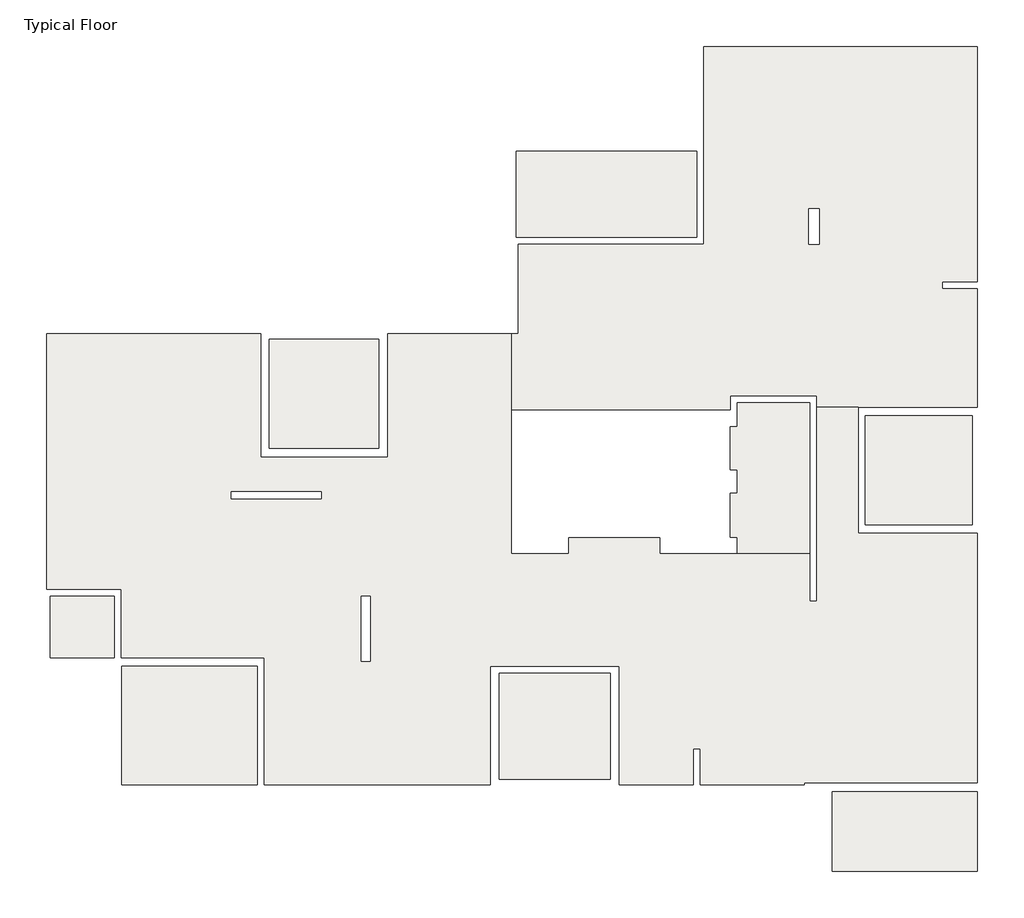
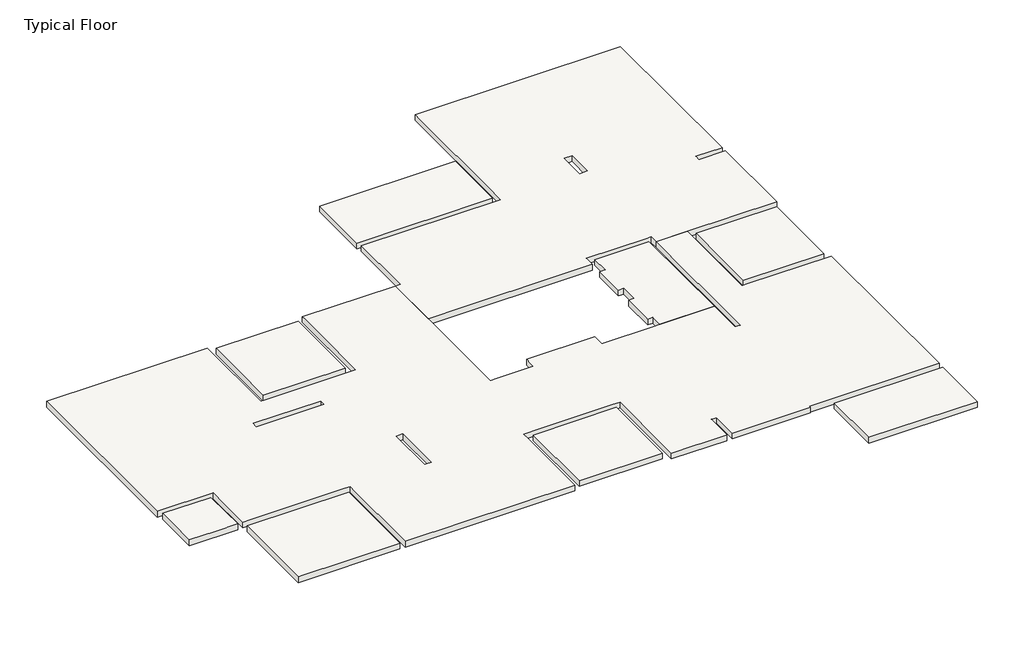
# One storey: 10 slabs.
"""IFC4 building model written with IfcOpenShell, lengths in millimetres."""

import ifcopenshell
import ifcopenshell.guid

model = None  # the IFC model being written
_history = None  # IfcOwnerHistory: only IFC2X3 demands one
_inside = {}  # id of a spatial element -> (the spatial element, [elements in it])
_under = {}  # id of a project, library or spatial element -> (it, [spatial elements below it])
_declared = {}  # id of a project -> (the project, [libraries it declares])
_typed = {}  # id of a type object -> (the type object, [elements of that type])
_made_of = {}  # id of a material, layer set ... -> (it, [elements and type objects made of it])


def new_model(schema):
    """Start an empty IFC model of exactly this schema.

    Asked for "IFC4X3", IfcOpenShell would pick the latest addendum, in which some entities
    have other attributes; the version numbers below select the first issue.
    IFC2X3 requires an IfcOwnerHistory on every rooted entity: one is made here for all.
    """
    global model, _history
    if schema == "IFC4X3":
        model = ifcopenshell.file(schema_version=(4, 3, 0, 0))
    else:
        model = ifcopenshell.file(schema=schema)
    _inside.clear()
    _under.clear()
    _declared.clear()
    _typed.clear()
    _made_of.clear()
    _history = None
    if model.schema == "IFC2X3":
        org = make("IfcOrganization", Name="unknown")
        user = make(
            "IfcPersonAndOrganization",
            ThePerson=make("IfcPerson", FamilyName="unknown"),
            TheOrganization=org,
        )
        app = make(
            "IfcApplication",
            ApplicationDeveloper=org,
            Version="unknown",
            ApplicationFullName="unknown",
            ApplicationIdentifier="unknown",
        )
        _history = make(
            "IfcOwnerHistory",
            OwningUser=user,
            OwningApplication=app,
            ChangeAction="ADDED",
            CreationDate=0,
        )
    return model


def make(cls, **values):
    """One entity of the class cls with the attributes given. An attribute that is None is left unset."""
    return model.create_entity(
        cls, **{name: value for name, value in values.items() if value is not None}
    )


def rooted(cls, **values):
    """An entity with a GlobalId (a new one), such as an element, a storey or a relation."""
    return make(cls, GlobalId=ifcopenshell.guid.new(), OwnerHistory=_history, **values)


def si_unit(unit_type, name, prefix=None):
    """IfcSIUnit, for example si_unit("LENGTHUNIT", "METRE", prefix="MILLI")."""
    return make("IfcSIUnit", UnitType=unit_type, Prefix=prefix, Name=name)


def assignment(units):
    """IfcUnitAssignment: the units of a project."""
    return None if units is None else make("IfcUnitAssignment", Units=units)


def point(xyz):
    """IfcCartesianPoint."""
    return None if xyz is None else make("IfcCartesianPoint", Coordinates=xyz)


def direction(xyz):
    """IfcDirection."""
    return None if xyz is None else make("IfcDirection", DirectionRatios=xyz)


def frame(location, z_axis=None, x_axis=None):
    """IfcAxis2Placement3D, a coordinate frame: its origin and axes. An axis left out is left unset."""
    return make(
        "IfcAxis2Placement3D",
        Location=point(location),
        Axis=direction(z_axis),
        RefDirection=direction(x_axis),
    )


def origin():
    """The frame at (0, 0, 0) with its axes left unset."""
    return frame((0.0, 0.0, 0.0))


def place(relative_to, where):
    """IfcLocalPlacement: puts the frame where relative to a parent placement (None: the world)."""
    return make(
        "IfcLocalPlacement", PlacementRelTo=relative_to, RelativePlacement=where
    )


def context(
    kind, dimensions, precision=None, world=None, true_north=None, identifier=None
):
    """IfcGeometricRepresentationContext, for example the 3D "Model" context."""
    return make(
        "IfcGeometricRepresentationContext",
        ContextIdentifier=identifier,
        ContextType=kind,
        CoordinateSpaceDimension=dimensions,
        Precision=precision,
        WorldCoordinateSystem=world,
        TrueNorth=true_north,
    )


def project(units=None, contexts=None):
    """IfcProject with its units and contexts."""
    return rooted(
        "IfcProject",
        Name="project",
        RepresentationContexts=contexts,
        UnitsInContext=assignment(units),
    )


def spatial(cls, under=None, at=None, **own):
    """A site, building, storey or space (cls), placed at a placement, below another one or the project."""
    s = rooted(cls, ObjectPlacement=at, **own)
    if under is not None:
        _under.setdefault(under.id(), (under, []))[1].append(s)
    return s


def polyline(points):
    """IfcPolyline through the points."""
    return make("IfcPolyline", Points=[point(p) for p in points])


def outline(outer, holes=None, kind="AREA"):
    """IfcArbitraryClosedProfileDef: a profile drawn as a closed curve; with holes, ...WithVoids."""
    if holes is None:
        return make("IfcArbitraryClosedProfileDef", ProfileType=kind, OuterCurve=outer)
    return make(
        "IfcArbitraryProfileDefWithVoids",
        ProfileType=kind,
        OuterCurve=outer,
        InnerCurves=holes,
    )


def extrude(swept, where, along, depth):
    """IfcExtrudedAreaSolid: the profile swept, set in the frame where, extruded along a direction by depth."""
    return make(
        "IfcExtrudedAreaSolid",
        SweptArea=swept,
        Position=where,
        ExtrudedDirection=direction(along),
        Depth=depth,
    )


def faces_of(points, faces, orient=None, outer=None):
    """IfcFace entities. A face is a list of loops; a loop is a list of indices into points, from 0.

    orient and outer hold one flag for each loop. By default every Orientation is true, the
    first loop of a face is its IfcFaceOuterBound and the others are IfcFaceBound.
    """
    made = []
    for i, loops in enumerate(faces):
        bounds = []
        for j, loop in enumerate(loops):
            is_outer = j == 0 if outer is None else outer[i][j]
            bounds.append(
                make(
                    "IfcFaceOuterBound" if is_outer else "IfcFaceBound",
                    Bound=make("IfcPolyLoop", Polygon=[points[k] for k in loop]),
                    Orientation=True if orient is None else orient[i][j],
                )
            )
        made.append(make("IfcFace", Bounds=bounds))
    return made


def faceted_brep(points, faces, orient=None, outer=None, voids=None):
    """IfcFacetedBrep: a solid bounded by flat faces; with voids (closed shells), ...WithVoids."""
    shared = [point(p) for p in points]
    hull = make("IfcClosedShell", CfsFaces=faces_of(shared, faces, orient, outer))
    if voids is None:
        return make("IfcFacetedBrep", Outer=hull)
    return make(
        "IfcFacetedBrepWithVoids",
        Outer=hull,
        Voids=[
            make(cls, CfsFaces=faces_of(shared, fs, o, b)) for cls, fs, o, b in voids
        ],
    )


def shape(context_of_items, identifier, shape_type, items):
    """IfcShapeRepresentation: the items that make up one representation, for example the "Body"."""
    return make(
        "IfcShapeRepresentation",
        ContextOfItems=context_of_items,
        RepresentationIdentifier=identifier,
        RepresentationType=shape_type,
        Items=items,
    )


def made_of(thing, what):
    """Note that an element or type object is made of a material, layer set ...; save() writes the relation."""
    if what is not None:
        _made_of.setdefault(what.id(), (what, []))[1].append(thing)
    return thing


def element(
    cls,
    number,
    at=None,
    inside=None,
    cuts=None,
    type_object=None,
    material=None,
    context=None,
    identifier="Body",
    shape_type=None,
    held_by="IfcProductDefinitionShape",
    body=None,
    shapes=None,
    **own,
):
    """One element of the class cls, such as IfcWall. Its Tag is "e" and its number.

    at: its placement. inside: the storey or other place that contains it. cuts: it is an
    opening in that element (IfcRelVoidsElement). A single representation is given by context,
    identifier, shape_type and body (its items); several are given by shapes. held_by: the class
    of the entity that holds the representations. save() writes the other relations.
    """
    e = rooted(cls, Tag="e%d" % number, ObjectPlacement=at, **own)
    if body is not None:
        shapes = [shape(context, identifier, shape_type, body)]
    if shapes is not None:
        e.Representation = make(held_by, Representations=shapes)
    if inside is not None:
        _inside.setdefault(inside.id(), (inside, []))[1].append(e)
    if cuts is not None:
        rooted(
            "IfcRelVoidsElement", RelatingBuildingElement=cuts, RelatedOpeningElement=e
        )
    if type_object is not None:
        _typed.setdefault(type_object.id(), (type_object, []))[1].append(e)
    return made_of(e, material)


def aggregate(whole, parts):
    """IfcRelAggregates: a whole, such as a stair, and the parts it consists of."""
    return rooted("IfcRelAggregates", RelatingObject=whole, RelatedObjects=parts)


def save(model, path):
    """Write the relations noted so far, then the file.

    IfcRelAggregates (storeys below a building ...), IfcRelContainedInSpatialStructure (elements
    in a storey), IfcRelDefinesByType, IfcRelAssociatesMaterial and IfcRelDeclares: one each for
    every whole, place, type object, material and project.
    """
    for whole, parts in _under.values():
        aggregate(whole, parts)
    for where, things in _inside.values():
        rooted(
            "IfcRelContainedInSpatialStructure",
            RelatedElements=things,
            RelatingStructure=where,
        )
    for kind, things in _typed.values():
        rooted("IfcRelDefinesByType", RelatedObjects=things, RelatingType=kind)
    for what, things in _made_of.values():
        rooted("IfcRelAssociatesMaterial", RelatedObjects=things, RelatingMaterial=what)
    for by, libraries in _declared.values():
        rooted("IfcRelDeclares", RelatingContext=by, RelatedDefinitions=libraries)
    model.write(path)


model = new_model("IFC4")

# Units and contexts
model_context = context("Model", 3, world=origin())
ifc_project = project(units=[si_unit("LENGTHUNIT", "METRE", prefix="MILLI")], contexts=[model_context])

# Site, building, storey
site = spatial("IfcSite", under=ifc_project)
building = spatial("IfcBuilding", under=site)
storey = spatial("IfcBuildingStorey", under=building, Name="Typical Floor", Elevation=3000.0)

# Slabs
placement = place(None, origin())
element("IfcSlab", 1, ObjectType="23", at=placement, inside=storey, context=model_context, shape_type="SweptSolid", body=[
    extrude(outline(polyline([(-1087.6785216, -1679.3693914), (-1087.6785216, -4688.4211868), (-4236.4747594, -4688.4211868), (-4236.4747594, -1679.3693914), (-1087.6785216, -1679.3693914)])), frame((0.0, 0.0, 2770.0), z_axis=(0.0, 0.0, 1.0), x_axis=(1.0, 0.0, 0.0)), (0.0, 0.0, 1.0), 230.0),
])
element("IfcSlab", 2, ObjectType="23", at=placement, inside=storey, context=model_context, shape_type="SweptSolid", body=[
    extrude(outline(polyline([(9307.3280344, -5038.4211868), (9307.3280344, -7293.4211868), (5207.3280344, -7293.4211868), (5207.3280344, -5038.4211868), (9307.3280344, -5038.4211868)])), frame((0.0, 0.0, 2770.0), z_axis=(0.0, 0.0, 1.0), x_axis=(1.0, 0.0, 0.0)), (0.0, 0.0, 1.0), 230.0),
])
element("IfcSlab", 3, ObjectType="23", at=placement, inside=storey, context=model_context, shape_type="SweptSolid", body=[
    extrude(outline(polyline([(-11093.5932474, -1488.4211868), (-11093.5932474, -4838.4211868), (-14933.5932474, -4838.4211868), (-14933.5932474, -1488.4211868), (-11093.5932474, -1488.4211868)])), frame((0.0, 0.0, 2770.0), z_axis=(0.0, 0.0, 1.0), x_axis=(1.0, 0.0, 0.0)), (0.0, 0.0, 1.0), 230.0),
])
element("IfcSlab", 4, ObjectType="23", at=placement, inside=storey, context=model_context, shape_type="Brep", body=[
    faceted_brep([(-15146.7835264, 502.021863, 2770.0), (-15146.7835264, -1238.4211868, 2770.0), (-16964.6329455, -1238.4211868, 2770.0), (-16964.6329455, 502.021863, 2770.0), (-15146.7835264, 502.021863, 3000.0), (-16964.6329455, 502.021863, 3000.0), (-16964.6329455, -228.1954104, 3000.0), (-16964.6329455, -1238.4211868, 3000.0), (-15973.5725457, -1238.4211868, 3000.0), (-15146.7835264, -1238.4211868, 3000.0)], [[[0, 1, 2, 3]], [[4, 5, 6, 7, 8, 9]], [[1, 0, 4, 9]], [[2, 1, 9, 8, 7]], [[3, 2, 7, 6, 5]], [[0, 3, 5, 4]]]),
])
element("IfcSlab", 5, ObjectType="23", at=placement, inside=storey, context=model_context, shape_type="SweptSolid", body=[
    extrude(outline(polyline([(-7647.5153815, 7788.5534768), (-7647.5153815, 4689.8992155), (-10746.4058847, 4689.8992155), (-10746.4058847, 7788.5534768), (-7647.5153815, 7788.5534768)])), frame((0.0, 0.0, 2770.0), z_axis=(0.0, 0.0, 1.0), x_axis=(1.0, 0.0, 0.0)), (0.0, 0.0, 1.0), 230.0),
])
element("IfcSlab", 6, ObjectType="23", at=placement, inside=storey, context=model_context, shape_type="SweptSolid", body=[
    extrude(outline(polyline([(9166.8868152, 5610.6924355), (9166.8868152, 2531.5477607), (6136.8868152, 2531.5477607), (6136.8868152, 5610.6924355), (9166.8868152, 5610.6924355)])), frame((0.0, 0.0, 2770.0), z_axis=(0.0, 0.0, 1.0), x_axis=(1.0, 0.0, 0.0)), (0.0, 0.0, 1.0), 230.0),
])
element("IfcSlab", 7, ObjectType="23", at=placement, inside=storey, context=model_context, shape_type="Brep", body=[
    faceted_brep([(-4486.4747594, -4838.4211868, 2770.0), (-10893.5932474, -4838.4211868, 2770.0), (-10893.5932474, -1238.4211868, 2770.0), (-11093.5932474, -1238.4211868, 2770.0), (-14946.7835264, -1238.4211868, 2770.0), (-14946.7835264, 701.4062462, 2770.0), (-14946.7835264, 702.021863, 2770.0), (-17064.6329455, 702.021863, 2770.0), (-17064.6329455, 7938.5534768, 2770.0), (-10996.4058847, 7938.5534768, 2770.0), (-10996.4058847, 4439.8992155, 2770.0), (-10746.4058847, 4439.8992155, 2770.0), (-7397.5153815, 4439.8992155, 2770.0), (-7397.5153815, 4689.8992155, 2770.0), (-7397.5153815, 7788.5534768, 2770.0), (-7397.5153815, 7938.5534768, 2770.0), (-3898.2455034, 7938.5534768, 2770.0), (-3898.2455034, 5780.7699278, 2770.0), (-3898.2455034, 5580.7699278, 2770.0), (-3898.2455034, 1710.8284517, 2770.0), (-3698.2455034, 1710.8284517, 2770.0), (-2268.2936764, 1710.8284517, 2770.0), (-2268.2936764, 1910.8284517, 2770.0), (-2268.2936764, 2161.3205984, 2770.0), (311.2984388, 2161.3205984, 2770.0), (311.2984388, 1910.8284517, 2770.0), (311.2984388, 1710.8284517, 2770.0), (2312.0172858, 1710.8284517, 2770.0), (2512.0172858, 1710.8284517, 2770.0), (4560.6810887, 1710.8284517, 2770.0), (4560.6810887, 359.9861346, 2770.0), (4760.6810887, 359.9861346, 2770.0), (4760.6810887, 5860.6924355, 2770.0), (5936.8868152, 5860.6924355, 2770.0), (5936.8868152, 5610.6924355, 2770.0), (5936.8868152, 2281.5477607, 2770.0), (6136.8868152, 2281.5477607, 2770.0), (9316.8868152, 2281.5477607, 2770.0), (9316.8868152, -4788.4211868, 2770.0), (4411.1547291, -4788.4211868, 2770.0), (4411.1547291, -4838.4211868, 2770.0), (1462.7563726, -4838.4211868, 2770.0), (1462.7563726, -3819.6429934, 2770.0), (1262.7563726, -3819.6429934, 2770.0), (1262.7563726, -4838.4211868, 2770.0), (-837.6785216, -4838.4211868, 2770.0), (-837.6785216, -1479.3693914, 2770.0), (-1087.6785216, -1479.3693914, 2770.0), (-4486.4747594, -1479.3693914, 2770.0), (-4486.4747594, -1679.3693914, 2770.0), (-7895.9524841, 504.5028364, 2770.0), (-8145.9524841, 504.5028364, 2770.0), (-8145.9524841, -1344.7765833, 2770.0), (-7895.9524841, -1344.7765833, 2770.0), (-11831.3488632, 3466.0170988, 2770.0), (-11831.3488632, 3266.0170988, 2770.0), (-9286.68122, 3266.0170988, 2770.0), (-9286.68122, 3466.0170988, 2770.0), (-10893.5932474, -4838.4211868, 3000.0), (-4486.4747594, -4838.4211868, 3000.0), (-4486.4747594, -1679.3693914, 3000.0), (-4486.4747594, -1479.3693914, 3000.0), (-1087.6785216, -1479.3693914, 3000.0), (-837.6785216, -1479.3693914, 3000.0), (-837.6785216, -4838.4211868, 3000.0), (1210.9852813, -4838.4211868, 3000.0), (1262.7563726, -4838.4211868, 3000.0), (1262.7563726, -3819.6429934, 3000.0), (1462.7563726, -3819.6429934, 3000.0), (1462.7563726, -4838.4211868, 3000.0), (4411.1547291, -4838.4211868, 3000.0), (4411.1547291, -4788.4211868, 3000.0), (9316.8868152, -4788.4211868, 3000.0), (9316.8868152, 2281.5477607, 3000.0), (6136.8868152, 2281.5477607, 3000.0), (5936.8868152, 2281.5477607, 3000.0), (5936.8868152, 5610.6924355, 3000.0), (5936.8868152, 5860.6924355, 3000.0), (4760.6810887, 5860.6924355, 3000.0), (4760.6810887, 359.9861346, 3000.0), (4560.6810887, 359.9861346, 3000.0), (4560.6810887, 1710.8284517, 3000.0), (2512.0172858, 1710.8284517, 3000.0), (2312.0172858, 1710.8284517, 3000.0), (311.2984388, 1710.8284517, 3000.0), (311.2984388, 1910.8284517, 3000.0), (311.2984388, 2161.3205984, 3000.0), (-2268.2936764, 2161.3205984, 3000.0), (-2268.2936764, 1910.8284517, 3000.0), (-2268.2936764, 1710.8284517, 3000.0), (-3698.2455034, 1710.8284517, 3000.0), (-3898.2455034, 1710.8284517, 3000.0), (-3898.2455034, 5580.7699278, 3000.0), (-3898.2455034, 5780.7699278, 3000.0), (-3898.2455034, 7938.5534768, 3000.0), (-7397.5153815, 7938.5534768, 3000.0), (-7397.5153815, 7788.5534768, 3000.0), (-7397.5153815, 4689.8992155, 3000.0), (-7397.5153815, 4439.8992155, 3000.0), (-10746.4058847, 4439.8992155, 3000.0), (-10996.4058847, 4439.8992155, 3000.0), (-10996.4058847, 7938.5534768, 3000.0), (-17064.6329455, 7938.5534768, 3000.0), (-17064.6329455, 702.021863, 3000.0), (-14946.7835264, 702.021863, 3000.0), (-14946.7835264, 701.4062462, 3000.0), (-14946.7835264, -1238.4211868, 3000.0), (-11093.5932474, -1238.4211868, 3000.0), (-10893.5932474, -1238.4211868, 3000.0), (-8145.9524841, 504.5028364, 3000.0), (-7895.9524841, 504.5028364, 3000.0), (-7895.9524841, -1344.7765833, 3000.0), (-8145.9524841, -1344.7765833, 3000.0), (-11831.3488632, 3266.0170988, 3000.0), (-11831.3488632, 3466.0170988, 3000.0), (-9286.68122, 3466.0170988, 3000.0), (-9286.68122, 3266.0170988, 3000.0)], [[[0, 1, 2, 3, 4, 5, 6, 7, 8, 9, 10, 11, 12, 13, 14, 15, 16, 17, 18, 19, 20, 21, 22, 23, 24, 25, 26, 27, 28, 29, 30, 31, 32, 33, 34, 35, 36, 37, 38, 39, 40, 41, 42, 43, 44, 45, 46, 47, 48, 49], [50, 51, 52, 53], [54, 55, 56, 57]], [[58, 59, 60, 61, 62, 63, 64, 65, 66, 67, 68, 69, 70, 71, 72, 73, 74, 75, 76, 77, 78, 79, 80, 81, 82, 83, 84, 85, 86, 87, 88, 89, 90, 91, 92, 93, 94, 95, 96, 97, 98, 99, 100, 101, 102, 103, 104, 105, 106, 107, 108], [109, 110, 111, 112], [113, 114, 115, 116]], [[1, 0, 59, 58]], [[2, 1, 58, 108]], [[2, 108, 107, 106, 4, 3]], [[4, 106, 105, 104, 6, 5]], [[7, 6, 104, 103]], [[8, 7, 103, 102]], [[9, 8, 102, 101]], [[10, 9, 101, 100]], [[10, 100, 99, 98, 12, 11]], [[12, 98, 97, 96, 95, 15, 14, 13]], [[16, 15, 95, 94]], [[17, 16, 94, 93]], [[17, 93, 92, 91, 19, 18]], [[19, 91, 90, 89, 21, 20]], [[21, 89, 88, 87, 23, 22]], [[24, 23, 87, 86]], [[24, 86, 85, 84, 26, 25]], [[26, 84, 83, 82, 81, 29, 28, 27]], [[30, 29, 81, 80]], [[31, 30, 80, 79]], [[32, 31, 79, 78]], [[33, 32, 78, 77]], [[33, 77, 76, 75, 35, 34]], [[35, 75, 74, 73, 37, 36]], [[38, 37, 73, 72]], [[39, 38, 72, 71]], [[40, 39, 71, 70]], [[41, 40, 70, 69]], [[42, 41, 69, 68]], [[43, 42, 68, 67]], [[44, 43, 67, 66]], [[45, 44, 66, 65, 64]], [[46, 45, 64, 63]], [[46, 63, 62, 61, 48, 47]], [[48, 61, 60, 59, 0, 49]], [[51, 50, 110, 109]], [[52, 51, 109, 112]], [[53, 52, 112, 111]], [[50, 53, 111, 110]], [[55, 54, 114, 113]], [[56, 55, 113, 116]], [[57, 56, 116, 115]], [[54, 57, 115, 114]]]),
])
element("IfcSlab", 8, ObjectType="23", at=placement, inside=storey, context=model_context, shape_type="Brep", body=[
    faceted_brep([(-3703.1131848, 10480.6924355, 2770.0), (1556.8868152, 10480.6924355, 2770.0), (1556.8868152, 10680.6924355, 2770.0), (1556.8868152, 16080.6924355, 2770.0), (9316.8868152, 16080.6924355, 2770.0), (9316.8868152, 9419.5945609, 2770.0), (8313.9644764, 9419.5945609, 2770.0), (8313.9644764, 9219.5945609, 2770.0), (9316.8868152, 9219.5945609, 2770.0), (9316.8868152, 5860.6924355, 2770.0), (5936.8868152, 5860.6924355, 2770.0), (4760.6810887, 5860.6924355, 2770.0), (4760.6810887, 6179.5864053, 2770.0), (4560.6810887, 6179.5864053, 2770.0), (2312.6329026, 6179.5864053, 2770.0), (2312.6329026, 5979.5864053, 2770.0), (2312.6329026, 5780.7699278, 2770.0), (-3898.2455034, 5780.7699278, 2770.0), (-3898.2455034, 7938.5534768, 2770.0), (-3703.1131848, 7938.5534768, 2770.0), (-3703.1131848, 8138.5534768, 2770.0), (4835.7759325, 11478.2299685, 2770.0), (4535.7759325, 11478.2299685, 2770.0), (4535.7759325, 10478.8270789, 2770.0), (4835.7759325, 10478.8270789, 2770.0), (1556.8868152, 10480.6924355, 3000.0), (-3703.1131848, 10480.6924355, 3000.0), (-3703.1131848, 8138.5534768, 3000.0), (-3703.1131848, 7938.5534768, 3000.0), (-3898.2455034, 7938.5534768, 3000.0), (-3898.2455034, 5780.7699278, 3000.0), (2312.6329026, 5780.7699278, 3000.0), (2312.6329026, 5979.5864053, 3000.0), (2312.6329026, 6179.5864053, 3000.0), (4560.6810887, 6179.5864053, 3000.0), (4760.6810887, 6179.5864053, 3000.0), (4760.6810887, 5860.6924355, 3000.0), (5936.8868152, 5860.6924355, 3000.0), (9316.8868152, 5860.6924355, 3000.0), (9316.8868152, 9219.5945609, 3000.0), (8313.9644764, 9219.5945609, 3000.0), (8313.9644764, 9419.5945609, 3000.0), (9316.8868152, 9419.5945609, 3000.0), (9316.8868152, 16080.6924355, 3000.0), (1556.8868152, 16080.6924355, 3000.0), (1556.8868152, 10680.6924355, 3000.0), (4535.7759325, 11478.2299685, 3000.0), (4835.7759325, 11478.2299685, 3000.0), (4835.7759325, 10478.8270789, 3000.0), (4535.7759325, 10478.8270789, 3000.0)], [[[0, 1, 2, 3, 4, 5, 6, 7, 8, 9, 10, 11, 12, 13, 14, 15, 16, 17, 18, 19, 20], [21, 22, 23, 24]], [[25, 26, 27, 28, 29, 30, 31, 32, 33, 34, 35, 36, 37, 38, 39, 40, 41, 42, 43, 44, 45], [46, 47, 48, 49]], [[26, 0, 20, 19, 28, 27]], [[1, 0, 26, 25]], [[1, 25, 45, 44, 3, 2]], [[4, 3, 44, 43]], [[5, 4, 43, 42]], [[6, 5, 42, 41]], [[7, 6, 41, 40]], [[8, 7, 40, 39]], [[9, 8, 39, 38]], [[9, 38, 37, 36, 11, 10]], [[12, 11, 36, 35]], [[12, 35, 34, 33, 14, 13]], [[14, 33, 32, 31, 16, 15]], [[17, 16, 31, 30]], [[18, 17, 30, 29]], [[19, 18, 29, 28]], [[22, 21, 47, 46]], [[23, 22, 46, 49]], [[24, 23, 49, 48]], [[21, 24, 48, 47]]]),
])
element("IfcSlab", 9, ObjectType="23", at=placement, inside=storey, context=model_context, shape_type="SweptSolid", body=[
    extrude(outline(polyline([(2512.0172858, 2179.3507401), (2312.6329026, 2179.3507401), (2312.6329026, 3415.5911695), (2512.0172858, 3415.5911695), (2512.0172858, 4085.9788147), (2312.6329026, 4085.9788147), (2312.6329026, 5304.757008), (2512.6329026, 5304.757008), (2512.6329026, 5979.5864053), (4560.6810887, 5979.5864053), (4560.6810887, 1710.8284517), (2512.0172858, 1710.8284517), (2512.0172858, 2179.3507401)])), frame((0.0, 0.0, 2770.0), z_axis=(0.0, 0.0, 1.0), x_axis=(1.0, 0.0, 0.0)), (0.0, 0.0, 1.0), 230.0),
])
element("IfcSlab", 10, ObjectType="23", at=placement, inside=storey, context=model_context, shape_type="Brep", body=[
    faceted_brep([(-3754.7272111, 10680.6924355, 2770.0), (-3754.7272111, 13112.8657791, 2770.0), (-3753.1131848, 13112.8657791, 2770.0), (1356.8868152, 13112.8657791, 2770.0), (1356.8868152, 13110.0948632, 2770.0), (1356.8868152, 10680.6924355, 2770.0), (-3753.1131848, 10680.6924355, 2770.0), (-3754.7272111, 13112.8657791, 3000.0), (-3754.7272111, 10680.6924355, 3000.0), (-3703.1131848, 10680.6924355, 3000.0), (1356.8868152, 10680.6924355, 3000.0), (1356.8868152, 13112.8657791, 3000.0), (-3753.1131848, 13112.8657791, 3000.0)], [[[0, 1, 2, 3, 4, 5, 6]], [[7, 8, 9, 10, 11, 12]], [[8, 0, 6, 5, 10, 9]], [[1, 0, 8, 7]], [[1, 7, 12, 11, 3, 2]], [[5, 4, 3, 11, 10]]]),
])

save(model, "model.ifc")

# Revit data of these elements
# Type "23"
#   Function = 0
#   Layers, outside or top first: 23 cm "Concrete" (function 1)
# Element 1 (IfcSlab, "23")
#   Mark = "S1"
#   SOFiSTiK_AMG_Comments = ""
#   Height Offset From Level = 0 cm
#   built-in parameter 1001954 = 1
#   SOFiSTiK_AMG_Scheduled = yes
#   SOFiSTiK_AMG_Adjusted = yes
#   Phase Created = New Construction
#   Materials on its faces: "Concrete"
# Element 2 (IfcSlab, "23")
#   Mark = "S2"
#   SOFiSTiK_AMG_Comments = ""
#   Height Offset From Level = 0 cm
#   built-in parameter 1001954 = 1
#   SOFiSTiK_AMG_Scheduled = yes
#   SOFiSTiK_AMG_Adjusted = yes
#   Phase Created = New Construction
#   Materials on its faces: "Concrete"
# Element 3 (IfcSlab, "23")
#   Mark = "S3"
#   SOFiSTiK_AMG_Comments = ""
#   Height Offset From Level = 0 cm
#   built-in parameter 1001954 = 1
#   SOFiSTiK_AMG_Scheduled = yes
#   SOFiSTiK_AMG_Adjusted = yes
#   Phase Created = New Construction
#   Materials on its faces: "Concrete"
# Element 4 (IfcSlab, "23")
#   Mark = "S4"
#   SOFiSTiK_AMG_Comments = ""
#   Height Offset From Level = 0 cm
#   built-in parameter 1001954 = 1
#   SOFiSTiK_AMG_Scheduled = yes
#   SOFiSTiK_AMG_Adjusted = yes
#   Phase Created = New Construction
#   Materials on its faces: "Concrete"
# Element 5 (IfcSlab, "23")
#   Mark = "S5"
#   SOFiSTiK_AMG_Comments = ""
#   Height Offset From Level = 0 cm
#   built-in parameter 1001954 = 1
#   SOFiSTiK_AMG_Scheduled = yes
#   SOFiSTiK_AMG_Adjusted = yes
#   Phase Created = New Construction
#   Materials on its faces: "Concrete"
# Element 6 (IfcSlab, "23")
#   Mark = "S6"
#   SOFiSTiK_AMG_Comments = ""
#   Height Offset From Level = 0 cm
#   built-in parameter 1001954 = 1
#   SOFiSTiK_AMG_Scheduled = yes
#   SOFiSTiK_AMG_Adjusted = yes
#   Phase Created = New Construction
#   Materials on its faces: "Concrete"
# Element 7 (IfcSlab, "23")
#   Mark = "S7"
#   SOFiSTiK_AMG_Comments = ""
#   Height Offset From Level = 0 cm
#   built-in parameter 1001954 = 1
#   SOFiSTiK_AMG_Scheduled = yes
#   SOFiSTiK_AMG_Adjusted = yes
#   Phase Created = New Construction
#   Materials on its faces: "Concrete"
# Element 8 (IfcSlab, "23")
#   Mark = "S8"
#   SOFiSTiK_AMG_Comments = ""
#   built-in parameter 1001955 = -1.5708 (stored number, unit not read)
#   Height Offset From Level = 0 cm
#   built-in parameter 1001954 = 1
#   SOFiSTiK_AMG_Scheduled = yes
#   SOFiSTiK_AMG_Adjusted = yes
#   Phase Created = New Construction
#   Materials on its faces: "Concrete"
# Element 9 (IfcSlab, "23")
#   Mark = "S9"
#   SOFiSTiK_AMG_Comments = ""
#   built-in parameter 1001955 = 1.5708 (stored number, unit not read)
#   Height Offset From Level = 0 cm
#   built-in parameter 1001954 = 1
#   SOFiSTiK_AMG_Scheduled = yes
#   SOFiSTiK_AMG_Adjusted = yes
#   Phase Created = New Construction
#   Materials on its faces: "Concrete"
# Element 10 (IfcSlab, "23")
#   Mark = "S10"
#   SOFiSTiK_AMG_Comments = ""
#   Height Offset From Level = 0 cm
#   built-in parameter 1001954 = 1
#   SOFiSTiK_AMG_Scheduled = yes
#   SOFiSTiK_AMG_Adjusted = yes
#   Phase Created = New Construction
#   Materials on its faces: "Concrete"
# Materials
#   "Concrete": class "Concrete", colour RGB 192 192 192, transparency 0, Keynote = "01000", Description = "Cast-in-place concrete", Cost = 0
